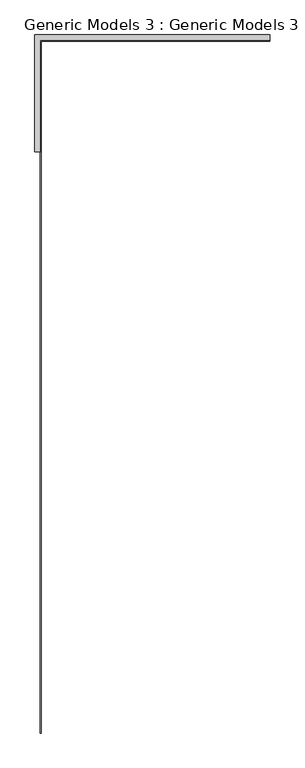
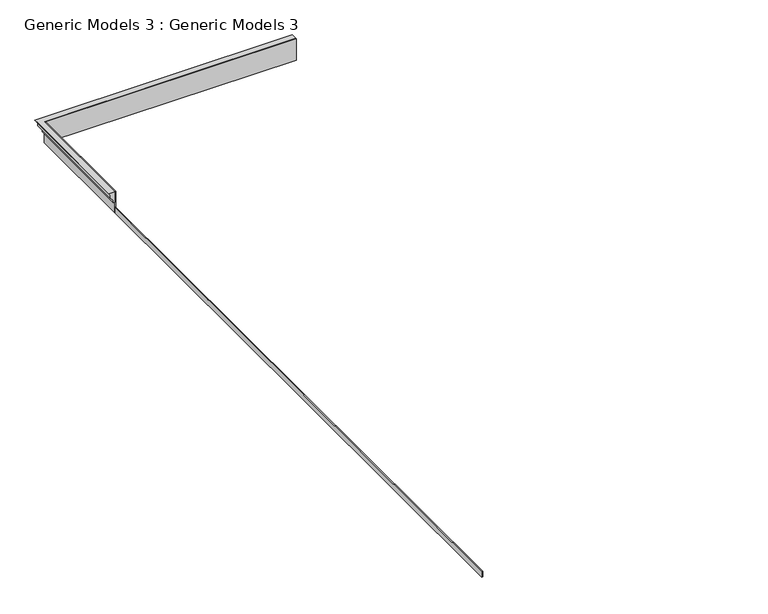
"""IFC4 building model written with IfcOpenShell, lengths in millimetres: proxy geometry, Generic Models 3 : Generic Models 3."""

from ifc_helpers import new_model, si_unit, frame, origin, place, context, project, spatial, polyline, outline, extrude, faceted_brep, source, transform, mapped, element, save


def generic_models_3_generic_models_3_5ee787fe(model_context):
    return source(origin(), model_context, "Body", "SolidModel", [
        faceted_brep([(25787.0402986, -22523.8830088, 3200.4), (25761.6402986, -22523.8830088, 3200.4), (25761.6402986, -22523.8830088, 3048.0), (25787.0402986, -22523.8830088, 3048.0), (25787.0402986, -5175.6830088, 3200.4), (25787.0402986, -5175.6830088, 3048.0), (25761.6402986, -5175.6830088, 3048.0), (25761.6402986, -5175.6830088, 3200.4), (25787.0402986, -14186.3330088, 3200.4), (25787.0402986, -14033.9330088, 3200.4), (25761.6402986, -14033.9330088, 3200.4), (25761.6402986, -14186.3330088, 3200.4), (25761.6402986, -14033.9330088, 3048.0), (25761.6402986, -14186.3330088, 3048.0), (25787.0402986, -14033.9330088, 3048.0), (25787.0402986, -14186.3330088, 3048.0)], [[[0, 1, 2, 3]], [[4, 5, 6, 7]], [[1, 0, 8, 9, 4, 7, 10, 11]], [[2, 1, 11, 10, 7, 6, 12, 13]], [[3, 2, 13, 12, 6, 5, 14, 15]], [[0, 3, 15, 14, 5, 4, 9, 8]]]),
        faceted_brep([(32629.1652986, -1810.1830088, 3352.8), (32629.1652986, -1810.1830088, 3422.65), (32629.1652986, -1729.3607037, 3503.4723051), (32629.1652986, -1729.3607037, 3592.3723051), (32629.1652986, -1683.68778, 3657.6), (32629.1652986, -1848.2830088, 3657.6), (32629.1652986, -1848.2830088, 3352.8), (25723.5402986, -1810.1830088, 3352.8), (25723.5402986, -1810.1830088, 3422.65), (25597.0450699, -1683.68778, 3657.6), (25597.0450699, -5175.6830088, 3657.6), (25761.6402986, -5175.6830088, 3657.6), (25761.6402986, -1848.2830088, 3657.6), (25761.6402986, -1848.2830088, 3352.8), (25761.6402986, -5175.6830088, 3352.8), (25723.5402986, -5175.6830088, 3352.8), (25642.7179935, -5175.6830088, 3592.3723051), (25642.7179935, -5175.6830088, 3503.4723051), (25723.5402986, -5175.6830088, 3422.65), (25642.7179935, -1729.3607037, 3503.4723051), (25642.7179935, -1729.3607037, 3592.3723051)], [[[0, 1, 2, 3, 4, 5, 6]], [[1, 0, 7, 8]], [[5, 4, 9, 10, 11, 12]], [[6, 5, 12, 13]], [[0, 6, 13, 14, 15, 7]], [[15, 14, 11, 10, 16, 17, 18]], [[8, 7, 15, 18]], [[13, 12, 11, 14]], [[2, 1, 8, 19]], [[3, 2, 19, 20]], [[4, 3, 20, 9]], [[19, 8, 18, 17]], [[20, 19, 17, 16]], [[9, 20, 16, 10]]]),
        extrude(outline(polyline([(32629.1652986, -1848.2830088), (32629.1652986, -1873.6830088), (25787.0402986, -1873.6830088), (25787.0402986, -5175.6830088), (25761.6402986, -5175.6830088), (25761.6402986, -1848.2830088), (32629.1652986, -1848.2830088)])), frame((0.0, 0.0, 3048.0), z_axis=(0.0, 0.0, 1.0), x_axis=(1.0, 0.0, 0.0)), (0.0, 0.0, 1.0), 609.6),
    ])


if __name__ == "__main__":
    model = new_model("IFC4")
    model_context = context("Model", 3, world=origin())
    ifc_project = project(units=[si_unit("LENGTHUNIT", "METRE", prefix="MILLI")], contexts=[model_context])
    site = spatial("IfcSite", under=ifc_project)
    building = spatial("IfcBuilding", under=site)
    placement = place(None, origin())
    generic_models_3_generic_models_3_shape = generic_models_3_generic_models_3_5ee787fe(model_context)
    element("IfcBuildingElementProxy", 1, Name="Generic Models 3 : Generic Models 3", ObjectType="Generic Models 3 : Generic Models 3", at=placement, inside=building, context=model_context, shape_type="MappedRepresentation", body=[
        mapped(generic_models_3_generic_models_3_shape, transform((0.0, 0.0, 0.0), x_axis=(1.0, 0.0, 0.0), y_axis=(0.0, 1.0, 0.0), z_axis=(0.0, 0.0, 1.0))),
    ])
    save(model, "model.ifc")

# Revit data of these elements
# Element 1 (IfcBuildingElementProxy, "Generic Models 3 : Generic Models 3")
#   Materials on its faces: "WHITE PAINT ON WOOD"
# Materials
#   "WHITE PAINT ON WOOD": class "Paint", colour RGB 255 255 255, transparency 0, Cost = 0
